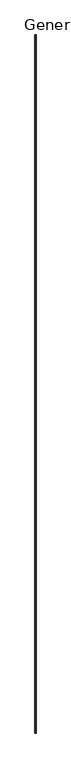
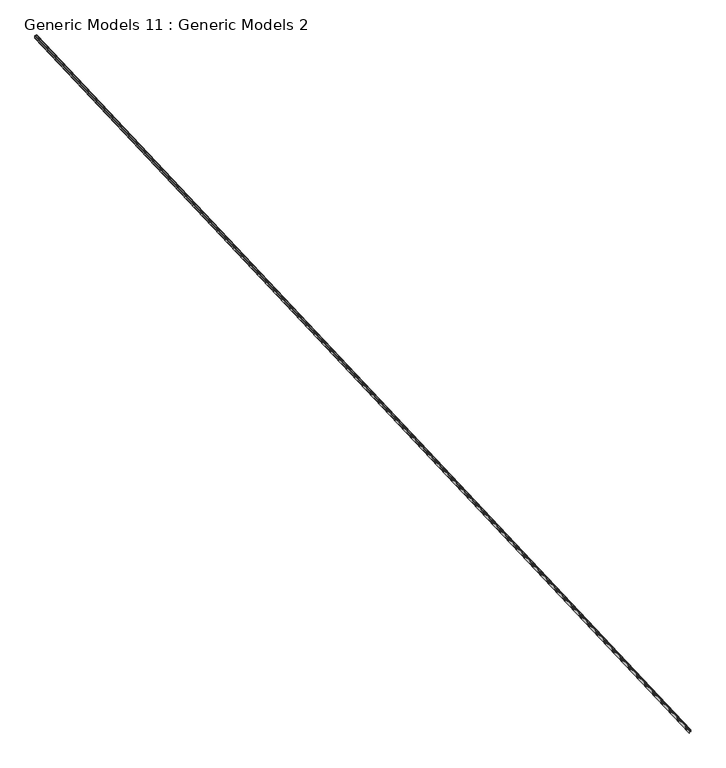
"""IFC4 building model written with IfcOpenShell, lengths in millimetres: proxy geometry, Generic Models 11 : Generic Models 2."""

from ifc_helpers import new_model, si_unit, frame, origin, place, context, project, spatial, polyline, outline, extrude, source, transform, mapped, element, save


def generic_models_11_generic_models_2_3684a208(model_context):
    return source(origin(), model_context, "Body", "SweptSolid", [
        extrude(outline(polyline([(-1.5874999, 0.0), (0.0, 0.0), (0.0, -2.7150899), (-71.9999999, -2.7150899), (-71.9999999, -1.1275899), (-70.4125, -1.1275899), (-70.4125, 49.6974101), (-71.9999999, 49.6974101), (-71.9999999, 51.2849101), (20.0, 51.2849101), (20.0, 42.8385386), (15.6126734, 42.8385386), (15.6126734, 44.4260386), (18.4125, 44.4260386), (18.4125, 49.6974101), (-1.5874999, 49.6974101), (-1.5874999, 42.8385386), (-5.9748265, 42.8385386), (-5.9748265, 44.4260386), (-3.175, 44.4260386), (-3.175, 49.6974101), (-54.6675027, 49.6974101), (-54.6675027, 21.2332689), (-68.8249999, 21.2332689), (-68.8249999, -1.1275899), (-1.5874999, -1.1275899), (-1.5874999, 0.0)]), holes=[polyline([(-61.7462514, 22.8207689), (-56.2550027, 22.8207689), (-56.2550027, 40.1667751), (-61.7462514, 40.1667751), (-61.7462514, 38.2413597), (-63.3337513, 38.2413597), (-63.3337513, 40.1667751), (-68.8249999, 40.1667751), (-68.8249999, 22.8207689), (-63.3337513, 22.8207689), (-63.3337513, 24.7461844), (-61.7462514, 24.7461844), (-61.7462514, 22.8207689)]), polyline([(-56.2550027, 49.6974101), (-68.8249999, 49.6974101), (-68.8249999, 41.7542751), (-56.2550027, 41.7542751), (-56.2550027, 49.6974101)])]), frame((667602.6423409, -569967.6846952, 8651.8737926), z_axis=(0.0, 0.9991330730923521, 0.041630544712176844), x_axis=(0.0, 0.041630544712176844, -0.9991330730923521)), (0.0, 0.0, 1.0), 33406.7702703),
    ])


if __name__ == "__main__":
    model = new_model("IFC4")
    model_context = context("Model", 3, world=origin())
    ifc_project = project(units=[si_unit("LENGTHUNIT", "METRE", prefix="MILLI")], contexts=[model_context])
    site = spatial("IfcSite", under=ifc_project)
    building = spatial("IfcBuilding", under=site)
    placement = place(None, origin())
    generic_models_11_generic_models_2_shape = generic_models_11_generic_models_2_3684a208(model_context)
    element("IfcBuildingElementProxy", 1, Name="Generic Models 11 : Generic Models 2", ObjectType="Generic Models 11 : Generic Models 2", at=placement, inside=building, context=model_context, shape_type="MappedRepresentation", body=[
        mapped(generic_models_11_generic_models_2_shape, transform((0.0, 0.0, 0.0), x_axis=(1.0, 0.0, 0.0), y_axis=(0.0, 1.0, 0.0), z_axis=(0.0, 0.0, 1.0))),
    ])
    save(model, "model.ifc")

# Revit data of these elements
# Element 1 (IfcBuildingElementProxy, "Generic Models 11 : Generic Models 2")
#   Materials on its faces: "THERMAL BROKEN ALUMINUM STOREFRONT FOR POLYCARBONATE"
# Materials
#   "THERMAL BROKEN ALUMINUM STOREFRONT FOR POLYCARBONATE": class "Unassigned", colour RGB 244 244 244, transparency 0, Keynote = "M07611300.01", Cost = 0
